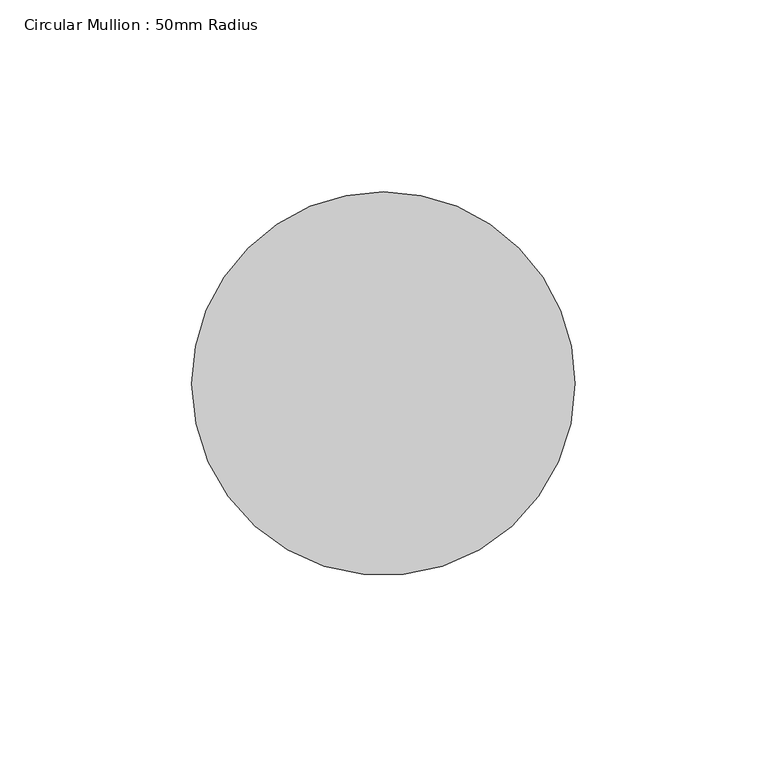
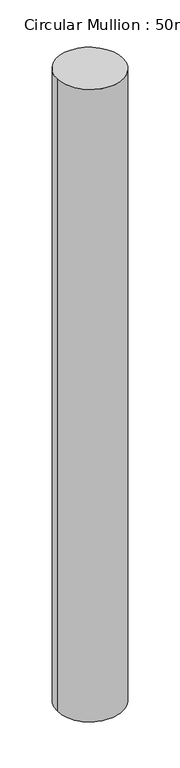
"""IFC4 building model written with IfcOpenShell, lengths in millimetres: member geometry, Circular Mullion : 50mm Radius."""

from ifc_helpers import new_model, si_unit, frame, origin, place, context, project, spatial, ellipse_curve, source, transform, mapped, element, save
from ifc_brep_helpers import plane_surface, cylinder_surface, advanced_brep


def circular_mullion_50mm_radius_72232090(model_context):
    return source(origin(), model_context, "Body", "AdvancedBrep", [
        advanced_brep(
        [(-100.0, 0.0, 1.6262085), (0.0, 0.0, 0.0), (0.0, 0.0, -1011.4204518), (-100.0, 0.0, -1013.0643779)],
        [
            (0, 1, ellipse_curve(frame((-50.0, 0.0, 0.8131042), z_axis=(-0.016258155714334064, -0.014793222441541007, -0.9997583872829294), x_axis=(-0.7394650917461505, -0.6728359465957666, 0.02198106133551768)), 50.0120836, 50.0)),
            (1, 2),
            (2, 3, ellipse_curve(frame((-50.0, 0.0, -1012.2424148), z_axis=(-0.016435202139413692, -0.01495431618395039, 0.9997530957982111), x_axis=(0.7394611779322713, 0.6728323854342366, 0.022220428481306363)), 50.0123483, 50.0)),
            (3, 0),
            (1, 0, ellipse_curve(frame((-50.0, 0.0, 0.8131042), z_axis=(-0.016258155714334064, -0.014793222441541007, -0.9997583872829294), x_axis=(-0.7394650917461505, -0.6728359465957666, 0.02198106133551768)), 50.0120836, 50.0)),
            (3, 2, ellipse_curve(frame((-50.0, 0.0, -1012.2424148), z_axis=(-0.016435202139413692, -0.01495431618395039, 0.9997530957982111), x_axis=(0.7394611779322713, 0.6728323854342366, 0.022220428481306363)), 50.0123483, 50.0)),
        ],
        [
            cylinder_surface(frame((-50.0, 0.0, 0.0), z_axis=(0.0, 0.0, 1.0), x_axis=(1.0, 0.0, 0.0)), 50.0),
            plane_surface(frame((-205.1299585, 225.44343, 0.0), z_axis=(0.016258155714334064, 0.014793222441541007, 0.9997583872829294), x_axis=(0.7394650917461502, 0.6728359465957667, -0.02198106133553259))),
            plane_surface(frame((-205.1299585, 225.44343, -1011.4204518), z_axis=(0.016435202139413692, 0.01495431618395039, -0.9997530957982111), x_axis=(0.7394611779322712, 0.6728323854342366, 0.022220428481308566))),
        ],
        [
            (0, [[1, 2, 3, 4]]),
            (0, [[5, -4, 6, -2]]),
            (1, [[-1, -5]]),
            (2, [[-6, -3]]),
        ],
    ),
    ])


if __name__ == "__main__":
    model = new_model("IFC4")
    model_context = context("Model", 3, world=origin())
    ifc_project = project(units=[si_unit("LENGTHUNIT", "METRE", prefix="MILLI")], contexts=[model_context])
    site = spatial("IfcSite", under=ifc_project)
    building = spatial("IfcBuilding", under=site)
    placement = place(None, origin())
    circular_mullion_50mm_radius_shape = circular_mullion_50mm_radius_72232090(model_context)
    element("IfcMember", 1, ObjectType="Circular Mullion : 50mm Radius", at=placement, inside=building, context=model_context, shape_type="MappedRepresentation", body=[
        mapped(circular_mullion_50mm_radius_shape, transform((0.0, 0.0, 0.0), x_axis=(1.0, 0.0, 0.0), y_axis=(0.0, 1.0, 0.0), z_axis=(0.0, 0.0, 1.0))),
    ])
    save(model, "model.ifc")

# Revit data of these elements
# Type "Circular Mullion : 50mm Radius"
#   built-in parameter 1007350 = 0.164042 (stored number, unit not read)
# Element 1 (IfcMember, "Circular Mullion : 50mm Radius")
#   Materials on its faces: "Aluminium"
# Materials
#   "Aluminium": class "Metal", colour RGB 247 247 247, transparency 0, Description = "Aluminium 6061", Cost = 0
